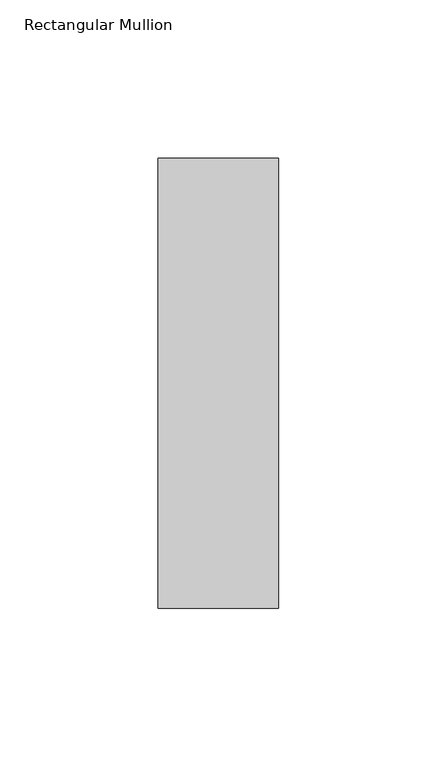
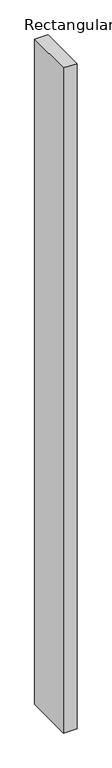
"""IFC4 building model written with IfcOpenShell, lengths in millimetres: member geometry, Rectangular Mullion : NLRS_21_CWM_hsb-regel 38x142_gen_rsf."""

from ifc_helpers import new_model, si_unit, frame, origin, place, context, project, spatial, polyline, outline, extrude, source, transform, mapped, element, save


def rectangular_mullion_69aae0b8(model_context):
    return source(origin(), model_context, "Body", "SweptSolid", [
        extrude(outline(polyline([(0.0, -71.0), (-38.0, -71.0), (-38.0, 71.0), (0.0, 71.0), (0.0, -71.0)])), frame((0.0, 0.0, -2000.0), z_axis=(0.0, 0.0, 1.0), x_axis=(1.0, 0.0, 0.0)), (0.0, 0.0, 1.0), 2000.0),
    ])


if __name__ == "__main__":
    model = new_model("IFC4")
    model_context = context("Model", 3, world=origin())
    ifc_project = project(units=[si_unit("LENGTHUNIT", "METRE", prefix="MILLI")], contexts=[model_context])
    site = spatial("IfcSite", under=ifc_project)
    building = spatial("IfcBuilding", under=site)
    placement = place(None, origin())
    rectangular_mullion_shape = rectangular_mullion_69aae0b8(model_context)
    element("IfcMember", 1, ObjectType="Rectangular Mullion : NLRS_21_CWM_hsb-regel 38x142_gen_rsf", at=placement, inside=building, context=model_context, shape_type="MappedRepresentation", body=[
        mapped(rectangular_mullion_shape, transform((0.0, 0.0, 0.0), x_axis=(1.0, 0.0, 0.0), y_axis=(0.0, 1.0, 0.0), z_axis=(0.0, 0.0, 1.0))),
    ])
    save(model, "model.ifc")

# Revit data of these elements
# Type "Rectangular Mullion : NLRS_21_CWM_hsb-regel 38x142_gen_rsf"
#   Export Type to IFC As = "IfcWall"
#   Type IfcGUID = "07M7mRoiH1CR8m_RSKIwpF"
#   Assembly Code = "21.10"
#   built-in parameter 1007322 = 0.465879 (stored number, unit not read)
#   built-in parameter 1007321 = 0.062336 (stored number, unit not read)
#   built-in parameter 1007320 = 0.062336 (stored number, unit not read)
# Element 1 (IfcMember, "Rectangular Mullion : NLRS_21_CWM_hsb-regel 38x142_gen_rsf")
#   Materials on its faces: "NLRS_i2_hout naaldhout vuren_gen_rsf"
# Materials
#   "NLRS_i2_hout naaldhout vuren_gen_rsf": class "I - Hout", colour RGB 234 199 147, transparency 0, Keynote = "i2", Manufacturer = "Revit Standards Foundation", URL = "www.revitstandards.org", Description = "hout vuren", Cost = 0
